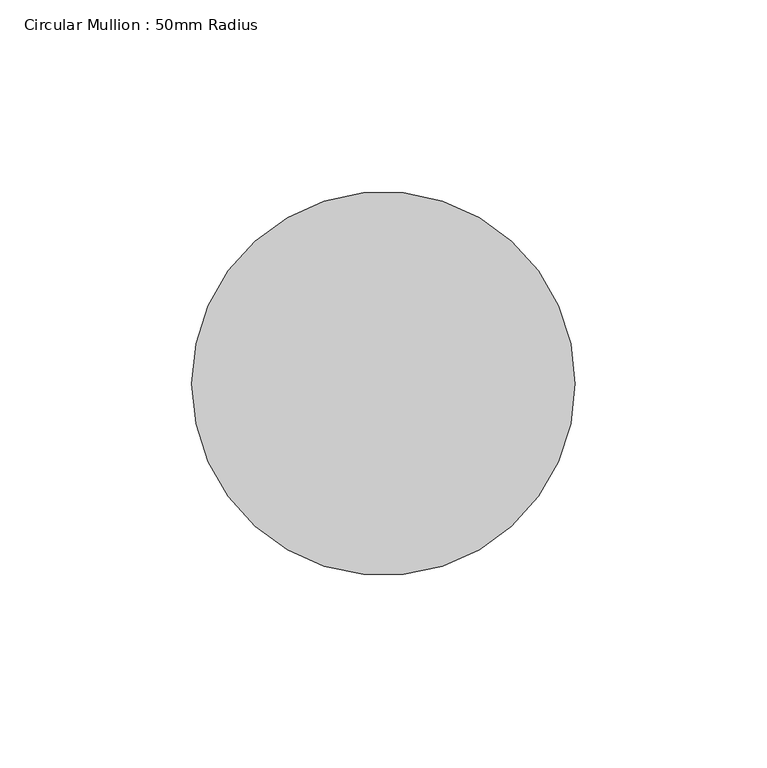
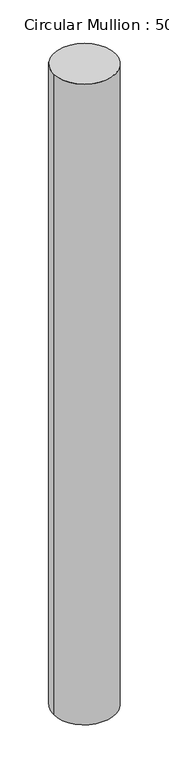
"""IFC4 building model written with IfcOpenShell, lengths in millimetres: member geometry, Circular Mullion : 50mm Radius."""

from ifc_helpers import new_model, si_unit, point, frame, origin, origin_2d, place, context, project, spatial, circle_curve, trimmed, segment, composite_curve, outline, extrude, source, transform, mapped, element, save


def circular_mullion_50mm_radius_15474724(model_context):
    return source(origin(), model_context, "Body", "SweptSolid", [
        extrude(outline(composite_curve([segment(trimmed(circle_curve(origin_2d(), 50.0), [point((50.0, 0.0))], [point((-50.0, 0.0))], False, "CARTESIAN"), True, "CONTINUOUS"), segment(trimmed(circle_curve(origin_2d(), 50.0), [point((-50.0, 0.0))], [point((50.0, 0.0))], False, "CARTESIAN"), True, "CONTINUOUS")], self_intersect=False)), frame((0.0, 0.0, -1093.4577414), z_axis=(0.0, 0.0, 1.0), x_axis=(1.0, 0.0, 0.0)), (0.0, 0.0, 1.0), 1093.4577414),
    ])


if __name__ == "__main__":
    model = new_model("IFC4")
    model_context = context("Model", 3, world=origin())
    ifc_project = project(units=[si_unit("LENGTHUNIT", "METRE", prefix="MILLI")], contexts=[model_context])
    site = spatial("IfcSite", under=ifc_project)
    building = spatial("IfcBuilding", under=site)
    placement = place(None, origin())
    circular_mullion_50mm_radius_shape = circular_mullion_50mm_radius_15474724(model_context)
    element("IfcMember", 1, ObjectType="Circular Mullion : 50mm Radius", at=placement, inside=building, context=model_context, shape_type="MappedRepresentation", body=[
        mapped(circular_mullion_50mm_radius_shape, transform((0.0, 0.0, 0.0), x_axis=(1.0, 0.0, 0.0), y_axis=(0.0, 1.0, 0.0), z_axis=(0.0, 0.0, 1.0))),
    ])
    save(model, "model.ifc")

# Revit data of these elements
# Type "Circular Mullion : 50mm Radius"
#   built-in parameter 1007350 = 0.164042 (stored number, unit not read)
# Element 1 (IfcMember, "Circular Mullion : 50mm Radius")
#   Materials on its faces: "Aluminium"
# Materials
#   "Aluminium": class "Metal", colour RGB 247 247 247, transparency 0, Description = "Aluminium 6061", Cost = 0
